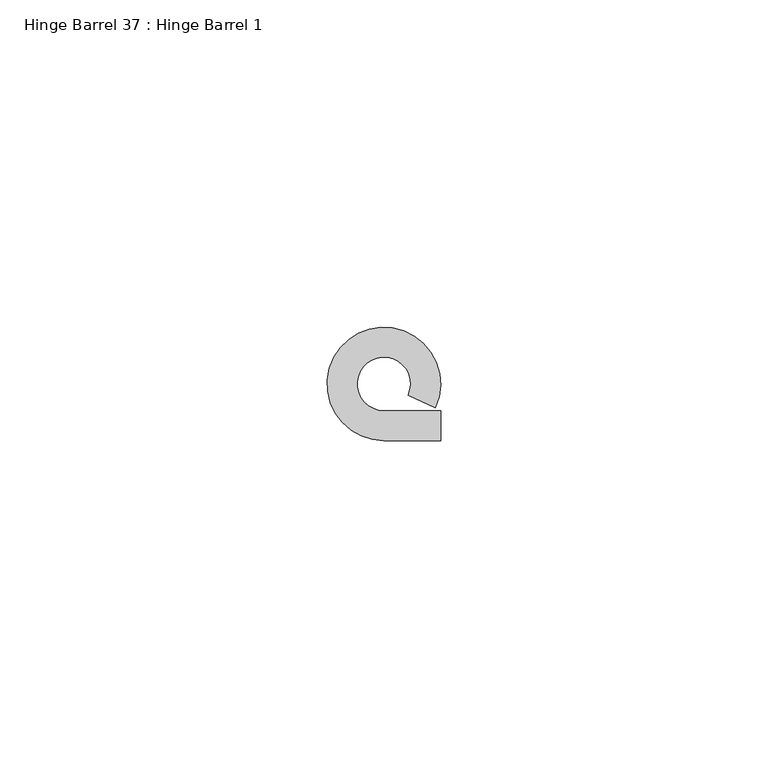
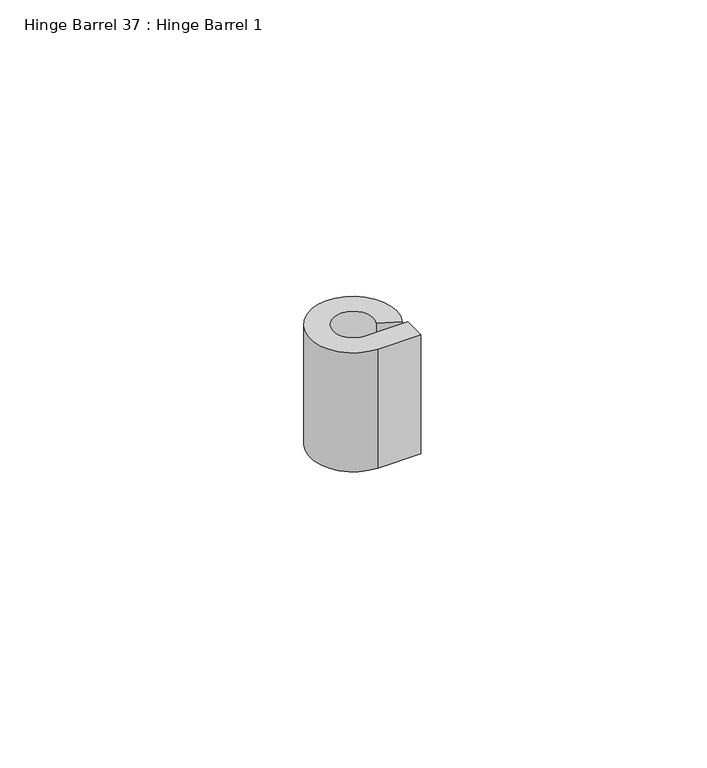
"""IFC4 building model written with IfcOpenShell, lengths in millimetres: proxy geometry, Hinge Barrel 37 : Hinge Barrel 1."""

from ifc_helpers import new_model, si_unit, point, frame, frame_2d, origin, place, context, project, spatial, polyline, circle_curve, trimmed, segment, composite_curve, outline, extrude, source, transform, mapped, element, save


def hinge_barrel_37_hinge_barrel_1_58d778a9(model_context):
    return source(origin(), model_context, "Body", "SweptSolid", [
        extrude(outline(composite_curve([segment(polyline([(587323.2214739, -534104.7943841), (587327.7934739, -534104.7943841), (587327.7934739, -534109.3584466), (587319.1320739, -534109.3584466)]), True, "CONTINUOUS"), segment(trimmed(circle_curve(frame_2d((587319.1320739, -534100.7049841)), 8.6534625), [point((587319.1320739, -534109.3584466))], [point((587326.986084, -534104.3377433))], False, "CARTESIAN"), True, "CONTINUOUS"), segment(polyline([(587326.986084, -534104.3377433), (587322.8436736, -534102.421731)]), True, "CONTINUOUS"), segment(trimmed(circle_curve(frame_2d((587319.1320739, -534100.7049841)), 4.0894), [point((587322.8436736, -534102.421731))], [point((587319.1320739, -534104.7943841))], True, "CARTESIAN"), True, "CONTINUOUS"), segment(polyline([(587319.1320739, -534104.7943841), (587323.2214739, -534104.7943841)]), True, "CONTINUOUS")], self_intersect=False)), frame((0.0, 0.0, 311.15), z_axis=(0.0, 0.0, 1.0), x_axis=(1.0, 0.0, 0.0)), (0.0, 0.0, 1.0), 25.4),
    ])


if __name__ == "__main__":
    model = new_model("IFC4")
    model_context = context("Model", 3, world=origin())
    ifc_project = project(units=[si_unit("LENGTHUNIT", "METRE", prefix="MILLI")], contexts=[model_context])
    site = spatial("IfcSite", under=ifc_project)
    building = spatial("IfcBuilding", under=site)
    placement = place(None, origin())
    hinge_barrel_37_hinge_barrel_1_shape = hinge_barrel_37_hinge_barrel_1_58d778a9(model_context)
    element("IfcBuildingElementProxy", 1, Name="Hinge Barrel 37 : Hinge Barrel 1", ObjectType="Hinge Barrel 37 : Hinge Barrel 1", at=placement, inside=building, context=model_context, shape_type="MappedRepresentation", body=[
        mapped(hinge_barrel_37_hinge_barrel_1_shape, transform((0.0, 0.0, 0.0), x_axis=(1.0, 0.0, 0.0), y_axis=(0.0, 1.0, 0.0), z_axis=(0.0, 0.0, 1.0))),
    ])
    save(model, "model.ifc")

# Revit data of these elements
# Element 1 (IfcBuildingElementProxy, "Hinge Barrel 37 : Hinge Barrel 1")
#   Materials on its faces: "6\"X6\" WELD-ON STL BUTT HINGE"
# Materials
#   "6\"X6\" WELD-ON STL BUTT HINGE": class "Metal", colour RGB 189 187 185, transparency 0, Description = "Carbon steel", Cost = 0
